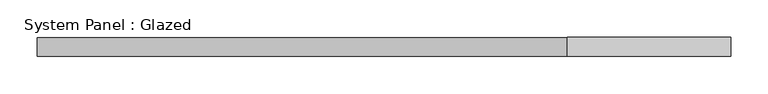
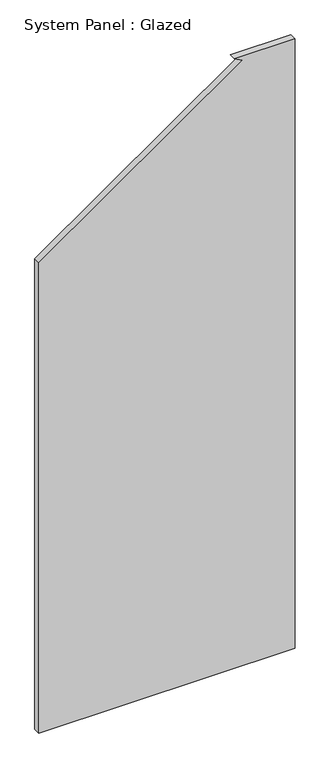
"""IFC4 building model written with IfcOpenShell, lengths in millimetres: plate geometry, System Panel : Glazed."""

from ifc_helpers import new_model, si_unit, frame, origin, place, context, project, spatial, polyline, outline, extrude, source, transform, mapped, element, save


def system_panel_glazed_8a08aa90(model_context):
    return source(origin(), model_context, "Body", "SweptSolid", [
        extrude(outline(polyline([(0.0, -462.5), (0.0, 462.5), (2325.0, 462.5), (2325.0, 244.388804), (2309.0423978, 273.0676259), (1793.9924013, -462.5), (0.0, -462.5)])), frame((0.0, 24.5, 0.0), z_axis=(0.0, 1.0, 0.0), x_axis=(0.0, 0.0, 1.0)), (0.0, 0.0, 1.0), 25.0),
    ])


if __name__ == "__main__":
    model = new_model("IFC4")
    model_context = context("Model", 3, world=origin())
    ifc_project = project(units=[si_unit("LENGTHUNIT", "METRE", prefix="MILLI")], contexts=[model_context])
    site = spatial("IfcSite", under=ifc_project)
    building = spatial("IfcBuilding", under=site)
    placement = place(None, origin())
    system_panel_glazed_shape = system_panel_glazed_8a08aa90(model_context)
    element("IfcPlate", 1, ObjectType="System Panel : Glazed", at=placement, inside=building, context=model_context, shape_type="MappedRepresentation", body=[
        mapped(system_panel_glazed_shape, transform((0.0, 0.0, 0.0), x_axis=(1.0, 0.0, 0.0), y_axis=(0.0, 1.0, 0.0), z_axis=(0.0, 0.0, 1.0))),
    ])
    save(model, "model.ifc")

# Revit data of these elements
# Type "System Panel : Glazed"
#   Construction Type Id = "GSP4R"
#   Analytic Construction = "1/8 in Pilkington single glazing"
#   Visual Light Transmittance = 0.9
#   Solar Heat Gain Coefficient = 0.86
#   Heat Transfer Coefficient (U) = 6.7069 W/(m²·K)
#   Define Thermal Properties by = 1
# Element 1 (IfcPlate, "System Panel : Glazed")
#   Materials on its faces: "Glass"
# Materials
#   "Glass": class "Glass", colour RGB 0 128 192, transparency 0.9, Description = "Soda Lime Glass", Cost = 0
